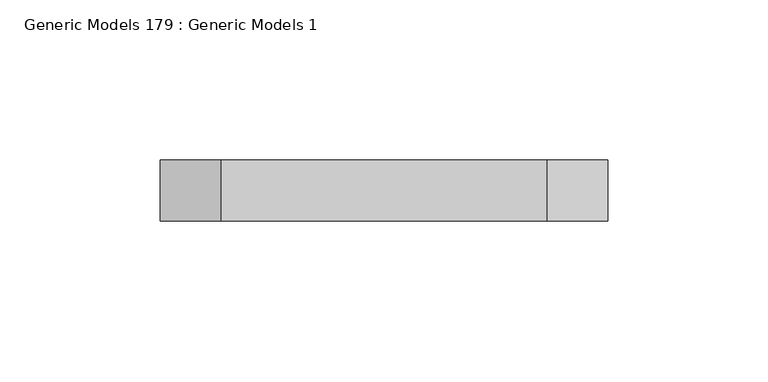
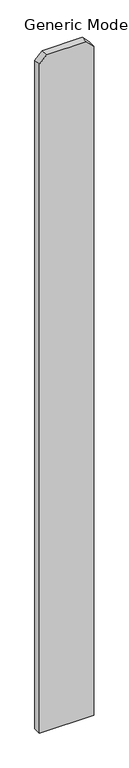
"""IFC4 building model written with IfcOpenShell, lengths in millimetres: proxy geometry, Generic Models 179 : Generic Models 1."""

import ifcopenshell
import ifcopenshell.guid

model = None  # the IFC model being written
_history = None  # IfcOwnerHistory: only IFC2X3 demands one
_inside = {}  # id of a spatial element -> (the spatial element, [elements in it])
_under = {}  # id of a project, library or spatial element -> (it, [spatial elements below it])
_declared = {}  # id of a project -> (the project, [libraries it declares])
_typed = {}  # id of a type object -> (the type object, [elements of that type])
_made_of = {}  # id of a material, layer set ... -> (it, [elements and type objects made of it])


def new_model(schema):
    """Start an empty IFC model of exactly this schema.

    Asked for "IFC4X3", IfcOpenShell would pick the latest addendum, in which some entities
    have other attributes; the version numbers below select the first issue.
    IFC2X3 requires an IfcOwnerHistory on every rooted entity: one is made here for all.
    """
    global model, _history
    if schema == "IFC4X3":
        model = ifcopenshell.file(schema_version=(4, 3, 0, 0))
    else:
        model = ifcopenshell.file(schema=schema)
    _inside.clear()
    _under.clear()
    _declared.clear()
    _typed.clear()
    _made_of.clear()
    _history = None
    if model.schema == "IFC2X3":
        org = make("IfcOrganization", Name="unknown")
        user = make(
            "IfcPersonAndOrganization",
            ThePerson=make("IfcPerson", FamilyName="unknown"),
            TheOrganization=org,
        )
        app = make(
            "IfcApplication",
            ApplicationDeveloper=org,
            Version="unknown",
            ApplicationFullName="unknown",
            ApplicationIdentifier="unknown",
        )
        _history = make(
            "IfcOwnerHistory",
            OwningUser=user,
            OwningApplication=app,
            ChangeAction="ADDED",
            CreationDate=0,
        )
    return model


def make(cls, **values):
    """One entity of the class cls with the attributes given. An attribute that is None is left unset."""
    return model.create_entity(
        cls, **{name: value for name, value in values.items() if value is not None}
    )


def rooted(cls, **values):
    """An entity with a GlobalId (a new one), such as an element, a storey or a relation."""
    return make(cls, GlobalId=ifcopenshell.guid.new(), OwnerHistory=_history, **values)


def si_unit(unit_type, name, prefix=None):
    """IfcSIUnit, for example si_unit("LENGTHUNIT", "METRE", prefix="MILLI")."""
    return make("IfcSIUnit", UnitType=unit_type, Prefix=prefix, Name=name)


def assignment(units):
    """IfcUnitAssignment: the units of a project."""
    return None if units is None else make("IfcUnitAssignment", Units=units)


def point(xyz):
    """IfcCartesianPoint."""
    return None if xyz is None else make("IfcCartesianPoint", Coordinates=xyz)


def direction(xyz):
    """IfcDirection."""
    return None if xyz is None else make("IfcDirection", DirectionRatios=xyz)


def frame(location, z_axis=None, x_axis=None):
    """IfcAxis2Placement3D, a coordinate frame: its origin and axes. An axis left out is left unset."""
    return make(
        "IfcAxis2Placement3D",
        Location=point(location),
        Axis=direction(z_axis),
        RefDirection=direction(x_axis),
    )


def origin():
    """The frame at (0, 0, 0) with its axes left unset."""
    return frame((0.0, 0.0, 0.0))


def place(relative_to, where):
    """IfcLocalPlacement: puts the frame where relative to a parent placement (None: the world)."""
    return make(
        "IfcLocalPlacement", PlacementRelTo=relative_to, RelativePlacement=where
    )


def context(
    kind, dimensions, precision=None, world=None, true_north=None, identifier=None
):
    """IfcGeometricRepresentationContext, for example the 3D "Model" context."""
    return make(
        "IfcGeometricRepresentationContext",
        ContextIdentifier=identifier,
        ContextType=kind,
        CoordinateSpaceDimension=dimensions,
        Precision=precision,
        WorldCoordinateSystem=world,
        TrueNorth=true_north,
    )


def project(units=None, contexts=None):
    """IfcProject with its units and contexts."""
    return rooted(
        "IfcProject",
        Name="project",
        RepresentationContexts=contexts,
        UnitsInContext=assignment(units),
    )


def spatial(cls, under=None, at=None, **own):
    """A site, building, storey or space (cls), placed at a placement, below another one or the project."""
    s = rooted(cls, ObjectPlacement=at, **own)
    if under is not None:
        _under.setdefault(under.id(), (under, []))[1].append(s)
    return s


def polyline(points):
    """IfcPolyline through the points."""
    return make("IfcPolyline", Points=[point(p) for p in points])


def outline(outer, holes=None, kind="AREA"):
    """IfcArbitraryClosedProfileDef: a profile drawn as a closed curve; with holes, ...WithVoids."""
    if holes is None:
        return make("IfcArbitraryClosedProfileDef", ProfileType=kind, OuterCurve=outer)
    return make(
        "IfcArbitraryProfileDefWithVoids",
        ProfileType=kind,
        OuterCurve=outer,
        InnerCurves=holes,
    )


def extrude(swept, where, along, depth):
    """IfcExtrudedAreaSolid: the profile swept, set in the frame where, extruded along a direction by depth."""
    return make(
        "IfcExtrudedAreaSolid",
        SweptArea=swept,
        Position=where,
        ExtrudedDirection=direction(along),
        Depth=depth,
    )


def shape(context_of_items, identifier, shape_type, items):
    """IfcShapeRepresentation: the items that make up one representation, for example the "Body"."""
    return make(
        "IfcShapeRepresentation",
        ContextOfItems=context_of_items,
        RepresentationIdentifier=identifier,
        RepresentationType=shape_type,
        Items=items,
    )


def source(mapping_origin, context_of_items, identifier, shape_type, items):
    """IfcRepresentationMap: a shape defined once, which mapped items show again and again."""
    return make(
        "IfcRepresentationMap",
        MappingOrigin=mapping_origin,
        MappedRepresentation=shape(context_of_items, identifier, shape_type, items),
    )


def transform(
    local_origin,
    x_axis=None,
    y_axis=None,
    z_axis=None,
    scale=None,
    scale2=None,
    scale3=None,
    uniform=True,
):
    """IfcCartesianTransformationOperator3D, or its non-uniform kind. x_axis, y_axis, z_axis: its Axis1, 2, 3."""
    if uniform:
        return make(
            "IfcCartesianTransformationOperator3D",
            Axis1=direction(x_axis),
            Axis2=direction(y_axis),
            LocalOrigin=point(local_origin),
            Scale=scale,
            Axis3=direction(z_axis),
        )
    return make(
        "IfcCartesianTransformationOperator3DnonUniform",
        Axis1=direction(x_axis),
        Axis2=direction(y_axis),
        LocalOrigin=point(local_origin),
        Scale=scale,
        Axis3=direction(z_axis),
        Scale2=scale2,
        Scale3=scale3,
    )


def mapped(mapping_source, mapping_target):
    """IfcMappedItem: shows the shape of a source again, moved by a transform."""
    return make(
        "IfcMappedItem", MappingSource=mapping_source, MappingTarget=mapping_target
    )


def made_of(thing, what):
    """Note that an element or type object is made of a material, layer set ...; save() writes the relation."""
    if what is not None:
        _made_of.setdefault(what.id(), (what, []))[1].append(thing)
    return thing


def element(
    cls,
    number,
    at=None,
    inside=None,
    cuts=None,
    type_object=None,
    material=None,
    context=None,
    identifier="Body",
    shape_type=None,
    held_by="IfcProductDefinitionShape",
    body=None,
    shapes=None,
    **own,
):
    """One element of the class cls, such as IfcWall. Its Tag is "e" and its number.

    at: its placement. inside: the storey or other place that contains it. cuts: it is an
    opening in that element (IfcRelVoidsElement). A single representation is given by context,
    identifier, shape_type and body (its items); several are given by shapes. held_by: the class
    of the entity that holds the representations. save() writes the other relations.
    """
    e = rooted(cls, Tag="e%d" % number, ObjectPlacement=at, **own)
    if body is not None:
        shapes = [shape(context, identifier, shape_type, body)]
    if shapes is not None:
        e.Representation = make(held_by, Representations=shapes)
    if inside is not None:
        _inside.setdefault(inside.id(), (inside, []))[1].append(e)
    if cuts is not None:
        rooted(
            "IfcRelVoidsElement", RelatingBuildingElement=cuts, RelatedOpeningElement=e
        )
    if type_object is not None:
        _typed.setdefault(type_object.id(), (type_object, []))[1].append(e)
    return made_of(e, material)


def aggregate(whole, parts):
    """IfcRelAggregates: a whole, such as a stair, and the parts it consists of."""
    return rooted("IfcRelAggregates", RelatingObject=whole, RelatedObjects=parts)


def save(model, path):
    """Write the relations noted so far, then the file.

    IfcRelAggregates (storeys below a building ...), IfcRelContainedInSpatialStructure (elements
    in a storey), IfcRelDefinesByType, IfcRelAssociatesMaterial and IfcRelDeclares: one each for
    every whole, place, type object, material and project.
    """
    for whole, parts in _under.values():
        aggregate(whole, parts)
    for where, things in _inside.values():
        rooted(
            "IfcRelContainedInSpatialStructure",
            RelatedElements=things,
            RelatingStructure=where,
        )
    for kind, things in _typed.values():
        rooted("IfcRelDefinesByType", RelatedObjects=things, RelatingType=kind)
    for what, things in _made_of.values():
        rooted("IfcRelAssociatesMaterial", RelatedObjects=things, RelatingMaterial=what)
    for by, libraries in _declared.values():
        rooted("IfcRelDeclares", RelatingContext=by, RelatedDefinitions=libraries)
    model.write(path)


def generic_models_179_generic_models_1_da8c2a58(model_context):
    return source(origin(), model_context, "Body", "SweptSolid", [
        extrude(outline(polyline([(76.2, 56970.6125), (1885.95, 56970.6125), (1905.0, 56951.5625), (1905.0, 56849.9625), (1885.95, 56830.9125), (76.2, 56830.9125), (76.2, 56970.6125)])), frame((0.0, 547.6875, 0.0), z_axis=(0.0, 1.0, 0.0), x_axis=(0.0, 0.0, 1.0)), (0.0, 0.0, 1.0), 19.05),
    ])


if __name__ == "__main__":
    model = new_model("IFC4")
    model_context = context("Model", 3, world=origin())
    ifc_project = project(units=[si_unit("LENGTHUNIT", "METRE", prefix="MILLI")], contexts=[model_context])
    site = spatial("IfcSite", under=ifc_project)
    building = spatial("IfcBuilding", under=site)
    placement = place(None, origin())
    generic_models_179_generic_models_1_shape = generic_models_179_generic_models_1_da8c2a58(model_context)
    element("IfcBuildingElementProxy", 1, Name="Generic Models 179 : Generic Models 1", ObjectType="Generic Models 179 : Generic Models 1", at=placement, inside=building, context=model_context, shape_type="MappedRepresentation", body=[
        mapped(generic_models_179_generic_models_1_shape, transform((0.0, 0.0, 0.0), x_axis=(1.0, 0.0, 0.0), y_axis=(0.0, 1.0, 0.0), z_axis=(0.0, 0.0, 1.0))),
    ])
    save(model, "model.ifc")

# Revit data of these elements
# Element 1 (IfcBuildingElementProxy, "Generic Models 179 : Generic Models 1")
#   Materials on its faces: "VERTICAL 1X6 CEDAR PLANKS W/ CLEAR WOOD SEALER"
# Materials
#   "VERTICAL 1X6 CEDAR PLANKS W/ CLEAR WOOD SEALER": class "Wood", colour RGB 234 198 147, transparency 0, Description = "Pinus Echinata", Cost = 0
